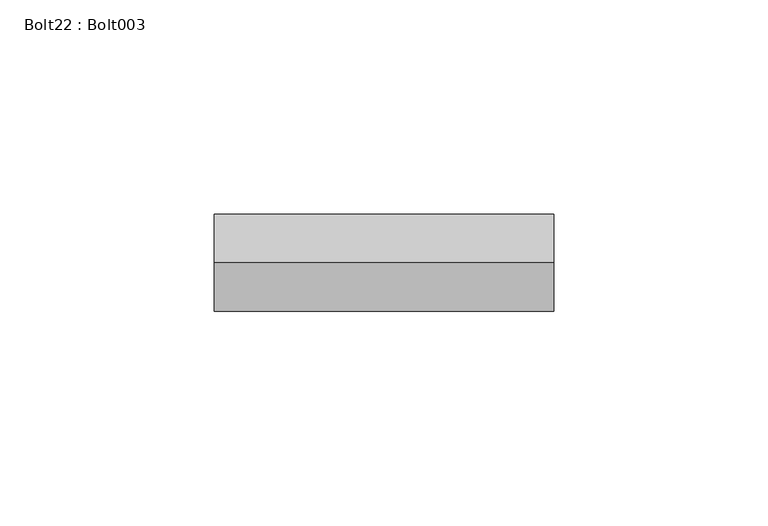
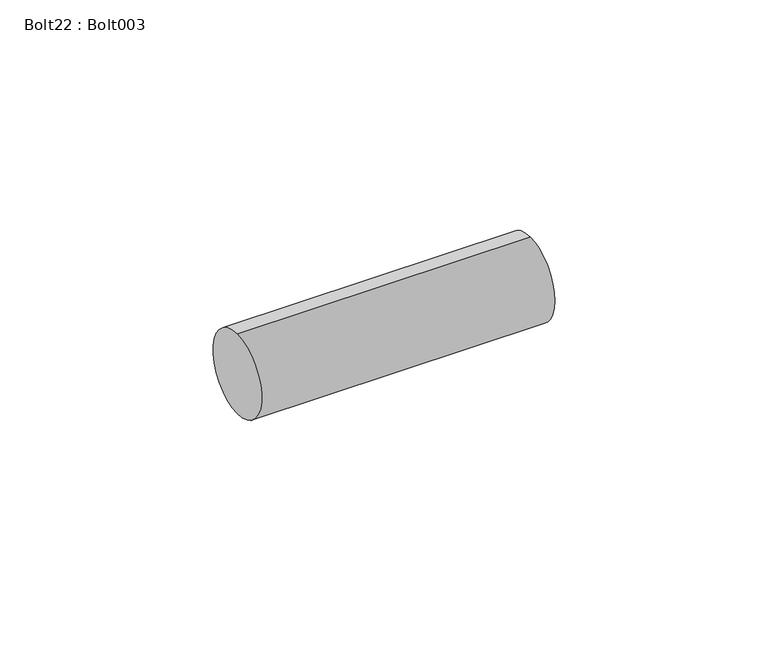
"""IFC4 building model written with IfcOpenShell, lengths in millimetres: proxy geometry, Bolt22 : Bolt003."""

from ifc_helpers import new_model, si_unit, point, frame, frame_2d, origin, place, context, project, spatial, circle_curve, trimmed, segment, composite_curve, outline, extrude, source, transform, mapped, element, save


def bolt22_bolt003_f2b5b441(model_context):
    return source(origin(), model_context, "Body", "SweptSolid", [
        extrude(outline(composite_curve([segment(trimmed(circle_curve(frame_2d((1985.8304801, 40070.0545241)), 11.4045168), [point((1985.8304801, 40058.6500073))], [point((1985.8304801, 40081.4590409))], False, "CARTESIAN"), True, "CONTINUOUS"), segment(trimmed(circle_curve(frame_2d((1985.8304801, 40070.0545241)), 11.4045168), [point((1985.8304801, 40081.4590409))], [point((1985.8304801, 40058.6500073))], False, "CARTESIAN"), True, "CONTINUOUS")], self_intersect=False)), frame((10265.0890809, 0.0, 0.0), z_axis=(1.0, 0.0, 0.0), x_axis=(0.0, 1.0, 0.0)), (0.0, 0.0, 1.0), 79.375),
    ])


if __name__ == "__main__":
    model = new_model("IFC4")
    model_context = context("Model", 3, world=origin())
    ifc_project = project(units=[si_unit("LENGTHUNIT", "METRE", prefix="MILLI")], contexts=[model_context])
    site = spatial("IfcSite", under=ifc_project)
    building = spatial("IfcBuilding", under=site)
    placement = place(None, origin())
    bolt22_bolt003_shape = bolt22_bolt003_f2b5b441(model_context)
    element("IfcBuildingElementProxy", 1, Name="Bolt22 : Bolt003", ObjectType="Bolt22 : Bolt003", at=placement, inside=building, context=model_context, shape_type="MappedRepresentation", body=[
        mapped(bolt22_bolt003_shape, transform((0.0, 0.0, 0.0), x_axis=(1.0, 0.0, 0.0), y_axis=(0.0, 1.0, 0.0), z_axis=(0.0, 0.0, 1.0))),
    ])
    save(model, "model.ifc")

# Revit data of these elements
# Type "Bolt22 : Bolt003"
#   NameOverride = "Bolt003"
# Element 1 (IfcBuildingElementProxy, "Bolt22 : Bolt003")
#   Materials on its faces: "TUBE STEEL STRINGER WELDED TO ANCHORED STEEL PLATE - SEE STRUCT DWGS"
# Materials
#   "TUBE STEEL STRINGER WELDED TO ANCHORED STEEL PLATE - SEE STRUCT DWGS": class "Unassigned", colour RGB 128 128 128, transparency 0, Cost = 0
